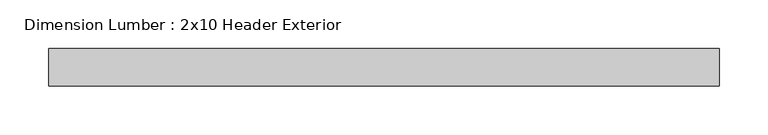
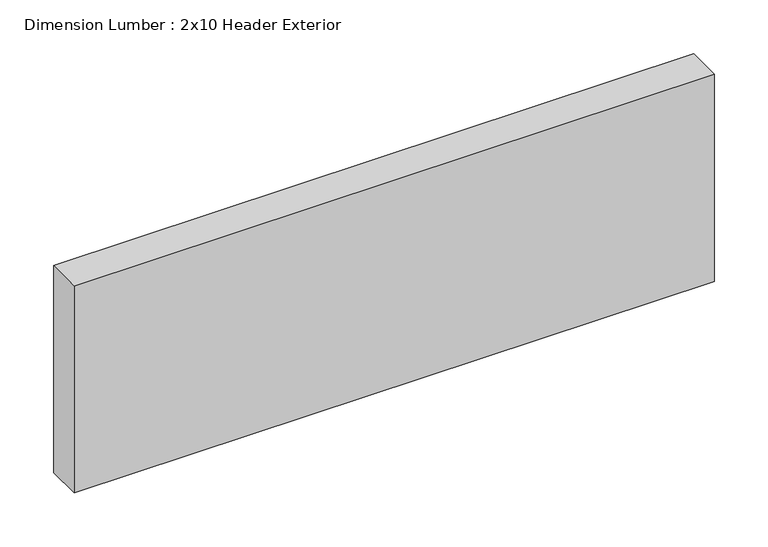
"""IFC4 building model written with IfcOpenShell, lengths in millimetres: beam geometry, Dimension Lumber : 2x10 Header Exterior."""

from ifc_helpers import new_model, si_unit, frame, origin, place, context, project, spatial, polyline, outline, extrude, source, transform, mapped, element, save


def dimension_lumber_2x10_header_exterior_80556d04(model_context):
    return source(origin(), model_context, "Body", "SweptSolid", [
        extrude(outline(polyline([(265.509375, 19.05), (265.509375, -19.05), (-420.290625, -19.05), (-420.290625, 19.05), (265.509375, 19.05)])), frame((0.0, 0.0, -117.475), z_axis=(0.0, 0.0, 1.0), x_axis=(1.0, 0.0, 0.0)), (0.0, 0.0, 1.0), 234.95),
    ])


if __name__ == "__main__":
    model = new_model("IFC4")
    model_context = context("Model", 3, world=origin())
    ifc_project = project(units=[si_unit("LENGTHUNIT", "METRE", prefix="MILLI")], contexts=[model_context])
    site = spatial("IfcSite", under=ifc_project)
    building = spatial("IfcBuilding", under=site)
    placement = place(None, origin())
    dimension_lumber_2x10_header_exterior_shape = dimension_lumber_2x10_header_exterior_80556d04(model_context)
    element("IfcBeam", 1, ObjectType="Dimension Lumber : 2x10 Header Exterior", at=placement, inside=building, context=model_context, shape_type="MappedRepresentation", body=[
        mapped(dimension_lumber_2x10_header_exterior_shape, transform((0.0, 0.0, 0.0), x_axis=(1.0, 0.0, 0.0), y_axis=(0.0, 1.0, 0.0), z_axis=(0.0, 0.0, 1.0))),
    ])
    save(model, "model.ifc")

# Revit data of these elements
# Type "Dimension Lumber : 2x10 Header Exterior"
#   Assembly Code = "B10"
#   A = 0.0963889 SF
#   Length [instance default] = 5' - 0"
#   b = 0' - 1 1/2"
#   d = 0' - 9 1/4"
#   Structural Material [instance default] = Softwood, Lumber
# Element 1 (IfcBeam, "Dimension Lumber : 2x10 Header Exterior")
#   Structural Material = Douglas Fir #2
#   Materials on its faces: "Douglas Fir #2"
# Materials
#   "Softwood, Lumber": class "Wood", colour RGB 223 192 134, transparency 0, Description = "Pinus Echinata", Cost = 0
#   "Douglas Fir #2": class "Wood", colour RGB 223 192 134, transparency 0, Description = "Pinus Echinata", Cost = 0
